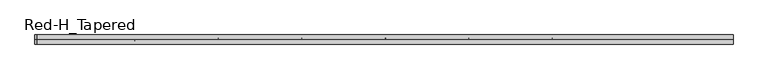
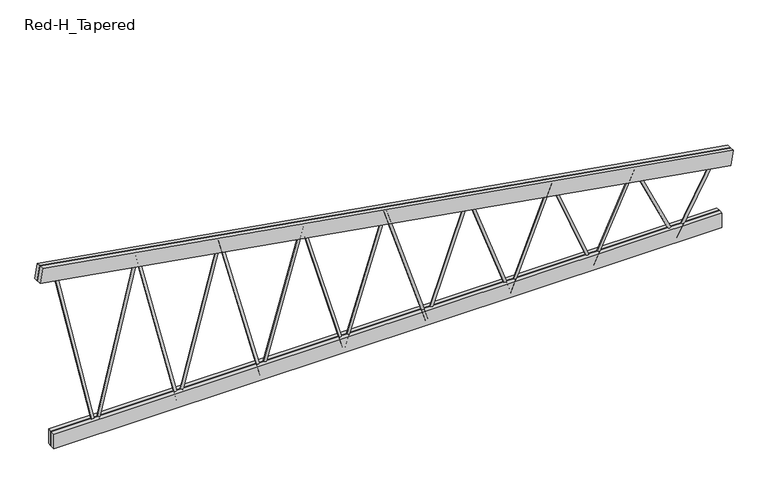
"""IFC4 building model written with IfcOpenShell, lengths in millimetres: beam geometry, Construction_Frames_RedBuilt_Openweb_Red-H_Tapered : Red-H_Tapered."""

from ifc_helpers import new_model, si_unit, point, frame, origin, origin_2d, place, context, project, spatial, polyline, circle_curve, trimmed, segment, composite_curve, outline, extrude, source, transform, mapped, element, save


def red_h_tapered_3aac71cb(model_context):
    return source(origin(), model_context, "Body", "SweptSolid", [
        extrude(outline(composite_curve([segment(trimmed(circle_curve(origin_2d(), 12.7), [point((0.0, -12.7))], [point((0.0, 12.7))], False, "CARTESIAN"), True, "CONTINUOUS"), segment(trimmed(circle_curve(origin_2d(), 12.7), [point((0.0, 12.7))], [point((0.0, -12.7))], False, "CARTESIAN"), True, "CONTINUOUS")], self_intersect=False)), frame((-378.61875, 0.0, -417.8101562), z_axis=(-0.277995532529411, 0.0, 0.9605823670532836), x_axis=(0.0, 1.0, 0.0)), (0.0, 0.0, 1.0), 1361.9598364),
        extrude(outline(composite_curve([segment(trimmed(circle_curve(origin_2d(), 12.7), [point((0.0, 12.7))], [point((0.0, -12.7))], False, "CARTESIAN"), True, "CONTINUOUS"), segment(trimmed(circle_curve(origin_2d(), 12.7), [point((0.0, -12.7))], [point((0.0, 12.7))], False, "CARTESIAN"), True, "CONTINUOUS")], self_intersect=False)), frame((-1135.85625, 0.0, -417.8101562), z_axis=(0.27799553252941006, 0.0, 0.9605823670532838), x_axis=(0.0, 1.0, 0.0)), (0.0, 0.0, 1.0), 1361.9598364),
        extrude(outline(composite_curve([segment(trimmed(circle_curve(origin_2d(), 12.7), [point((0.0, -12.7))], [point((0.0, 12.7000001))], False, "CARTESIAN"), True, "CONTINUOUS"), segment(trimmed(circle_curve(origin_2d(), 12.7), [point((0.0, 12.7000001))], [point((0.0, -12.7))], False, "CARTESIAN"), True, "CONTINUOUS")], self_intersect=False)), frame((-1135.85625, 0.0, -417.8101562), z_axis=(-0.2554865755688276, 0.0, 0.966812603198838), x_axis=(0.0, 1.0, 0.0)), (0.0, 0.0, 1.0), 1481.9516413),
        extrude(outline(composite_curve([segment(trimmed(circle_curve(origin_2d(), 12.7), [point((0.0, 12.7))], [point((0.0, -12.7000001))], False, "CARTESIAN"), True, "CONTINUOUS"), segment(trimmed(circle_curve(origin_2d(), 12.7), [point((0.0, -12.7000001))], [point((0.0, 12.7))], False, "CARTESIAN"), True, "CONTINUOUS")], self_intersect=False)), frame((-1893.09375, 0.0, -417.8101562), z_axis=(0.25548657556883586, 0.0, 0.9668126031988359), x_axis=(0.0, 1.0, 0.0)), (0.0, 0.0, 1.0), 1481.9516413),
        extrude(outline(composite_curve([segment(trimmed(circle_curve(origin_2d(), 12.7), [point((0.0, -12.7))], [point((0.0, 12.7))], False, "CARTESIAN"), True, "CONTINUOUS"), segment(trimmed(circle_curve(origin_2d(), 12.7), [point((0.0, 12.7))], [point((0.0, -12.7))], False, "CARTESIAN"), True, "CONTINUOUS")], self_intersect=False)), frame((-1893.09375, 0.0, -417.8101562), z_axis=(-0.23624830304325084, 0.0, 0.9716927185634275), x_axis=(0.0, 1.0, 0.0)), (0.0, 0.0, 1.0), 1602.6305591),
        extrude(outline(composite_curve([segment(trimmed(circle_curve(origin_2d(), 12.7), [point((0.0, 12.7))], [point((0.0, -12.7))], False, "CARTESIAN"), True, "CONTINUOUS"), segment(trimmed(circle_curve(origin_2d(), 12.7), [point((0.0, -12.7))], [point((0.0, 12.7))], False, "CARTESIAN"), True, "CONTINUOUS")], self_intersect=False)), frame((-2650.33125, 0.0, -417.8101562), z_axis=(0.23624830304324398, 0.0, 0.9716927185634292), x_axis=(0.0, 1.0, 0.0)), (0.0, 0.0, 1.0), 1602.6305591),
        extrude(outline(composite_curve([segment(trimmed(circle_curve(origin_2d(), 12.7), [point((0.0, -12.7))], [point((0.0, 12.7))], False, "CARTESIAN"), True, "CONTINUOUS"), segment(trimmed(circle_curve(origin_2d(), 12.7), [point((0.0, 12.7))], [point((0.0, -12.7))], False, "CARTESIAN"), True, "CONTINUOUS")], self_intersect=False)), frame((-2650.33125, 0.0, -417.8101562), z_axis=(-0.21963526223165897, 0.0, 0.9755820578426145), x_axis=(0.0, 1.0, 0.0)), (0.0, 0.0, 1.0), 1723.8522911),
        extrude(outline(composite_curve([segment(trimmed(circle_curve(origin_2d(), 12.7), [point((0.0, -12.7))], [point((0.0, 12.7))], False, "CARTESIAN"), True, "CONTINUOUS"), segment(trimmed(circle_curve(origin_2d(), 12.7), [point((0.0, 12.7))], [point((0.0, -12.7))], False, "CARTESIAN"), True, "CONTINUOUS")], self_intersect=False)), frame((2650.33125, 0.0, -417.8101562), z_axis=(0.48331839774277513, 0.0, 0.8754446449681195), x_axis=(0.0, 1.0, 0.0)), (0.0, 0.0, 1.0), 783.3733451),
        extrude(outline(composite_curve([segment(trimmed(circle_curve(origin_2d(), 12.7), [point((0.0, 12.7))], [point((0.0, -12.7))], False, "CARTESIAN"), True, "CONTINUOUS"), segment(trimmed(circle_curve(origin_2d(), 12.7), [point((0.0, -12.7))], [point((0.0, 12.7))], False, "CARTESIAN"), True, "CONTINUOUS")], self_intersect=False)), frame((2650.33125, 0.0, -417.8101562), z_axis=(-0.4233271479189003, 0.0, 0.9059768903426011), x_axis=(0.0, 1.0, 0.0)), (0.0, 0.0, 1.0), 894.3880681),
        extrude(outline(composite_curve([segment(trimmed(circle_curve(origin_2d(), 12.7), [point((0.0, -12.7))], [point((0.0, 12.7))], False, "CARTESIAN"), True, "CONTINUOUS"), segment(trimmed(circle_curve(origin_2d(), 12.7), [point((0.0, 12.7))], [point((0.0, -12.7))], False, "CARTESIAN"), True, "CONTINUOUS")], self_intersect=False)), frame((1893.09375, 0.0, -417.8101562), z_axis=(0.42332714791889964, 0.0, 0.9059768903426014), x_axis=(0.0, 1.0, 0.0)), (0.0, 0.0, 1.0), 894.3880681),
        extrude(outline(composite_curve([segment(trimmed(circle_curve(origin_2d(), 12.7), [point((0.0, 12.7))], [point((0.0, -12.7))], False, "CARTESIAN"), True, "CONTINUOUS"), segment(trimmed(circle_curve(origin_2d(), 12.7), [point((0.0, -12.7))], [point((0.0, 12.7))], False, "CARTESIAN"), True, "CONTINUOUS")], self_intersect=False)), frame((1893.09375, 0.0, -417.8101562), z_axis=(-0.3754069541599523, 0.0, 0.9268600858642838), x_axis=(0.0, 1.0, 0.0)), (0.0, 0.0, 1.0), 1008.5555044),
        extrude(outline(composite_curve([segment(trimmed(circle_curve(origin_2d(), 12.7), [point((0.0, -12.7))], [point((0.0, 12.7))], False, "CARTESIAN"), True, "CONTINUOUS"), segment(trimmed(circle_curve(origin_2d(), 12.7), [point((0.0, 12.7))], [point((0.0, -12.7))], False, "CARTESIAN"), True, "CONTINUOUS")], self_intersect=False)), frame((1135.85625, 0.0, -417.8101562), z_axis=(0.37540695415995146, 0.0, 0.9268600858642841), x_axis=(0.0, 1.0, 0.0)), (0.0, 0.0, 1.0), 1008.5555044),
        extrude(outline(composite_curve([segment(trimmed(circle_curve(origin_2d(), 12.7), [point((0.0, 12.7))], [point((0.0, -12.7))], False, "CARTESIAN"), True, "CONTINUOUS"), segment(trimmed(circle_curve(origin_2d(), 12.7), [point((0.0, -12.7))], [point((0.0, 12.7))], False, "CARTESIAN"), True, "CONTINUOUS")], self_intersect=False)), frame((1135.85625, 0.0, -417.8101562), z_axis=(-0.3365750833372033, 0.0, 0.9416566323647674), x_axis=(0.0, 1.0, 0.0)), (0.0, 0.0, 1.0), 1124.9161591),
        extrude(outline(composite_curve([segment(trimmed(circle_curve(origin_2d(), 12.7), [point((0.0, -12.7))], [point((0.0, 12.7))], False, "CARTESIAN"), True, "CONTINUOUS"), segment(trimmed(circle_curve(origin_2d(), 12.7), [point((0.0, 12.7))], [point((0.0, -12.7))], False, "CARTESIAN"), True, "CONTINUOUS")], self_intersect=False)), frame((378.61875, 0.0, -417.8101562), z_axis=(0.33657508333720376, 0.0, 0.9416566323647673), x_axis=(0.0, 1.0, 0.0)), (0.0, 0.0, 1.0), 1124.9161591),
        extrude(outline(composite_curve([segment(trimmed(circle_curve(origin_2d(), 12.7), [point((0.0, 12.7))], [point((0.0, -12.6999999))], False, "CARTESIAN"), True, "CONTINUOUS"), segment(trimmed(circle_curve(origin_2d(), 12.7), [point((0.0, -12.6999999))], [point((0.0, 12.7))], False, "CARTESIAN"), True, "CONTINUOUS")], self_intersect=False)), frame((378.61875, 0.0, -417.8101562), z_axis=(-0.3046365038173337, 0.0, 0.952468687433845), x_axis=(0.0, 1.0, 0.0)), (0.0, 0.0, 1.0), 1242.8541729),
        extrude(outline(composite_curve([segment(trimmed(circle_curve(origin_2d(), 12.7), [point((0.0, 12.6999999))], [point((0.0, -12.7))], False, "CARTESIAN"), True, "CONTINUOUS"), segment(trimmed(circle_curve(origin_2d(), 12.7), [point((0.0, -12.7))], [point((0.0, 12.6999999))], False, "CARTESIAN"), True, "CONTINUOUS")], self_intersect=False)), frame((-378.61875, 0.0, -417.8101562), z_axis=(0.30463650381731205, 0.0, 0.952468687433852), x_axis=(0.0, 1.0, 0.0)), (0.0, 0.0, 1.0), 1242.8541729),
        extrude(outline(polyline([(-3054.35, 41.275), (3054.35, 41.275), (3054.35, 3.175), (-3054.35, 3.175), (-3054.35, 41.275)])), frame((0.0, 0.0, -436.8601562), z_axis=(0.0, 0.0, 1.0), x_axis=(1.0, 0.0, 0.0)), (0.0, 0.0, 1.0), 139.7),
        extrude(outline(polyline([(-3054.35, -3.175), (3054.35, -3.175), (3054.35, -41.275), (-3054.35, -41.275), (-3054.35, -3.175)])), frame((0.0, 0.0, -436.8601562), z_axis=(0.0, 0.0, 1.0), x_axis=(1.0, 0.0, 0.0)), (0.0, 0.0, 1.0), 139.7),
        extrude(outline(polyline([(0.0, 38.1), (6401.4173313, 38.1), (6401.4173313, 0.0), (0.0, 0.0), (0.0, 38.1)])), frame((-3179.231088, 3.175, 1203.3934066), z_axis=(0.1666505938890901, 0.0, 0.9860160138437984), x_axis=(0.9860160138437984, 0.0, -0.1666505938890901)), (0.0, 0.0, 1.0), 139.7),
        extrude(outline(polyline([(0.0, 38.1), (6401.4173313, 38.1), (6401.4173313, 0.0), (0.0, 0.0), (0.0, 38.1)])), frame((-3179.231088, -41.275, 1203.3934066), z_axis=(0.1666505938890901, 0.0, 0.9860160138437984), x_axis=(0.9860160138437984, 0.0, -0.1666505938890901)), (0.0, 0.0, 1.0), 139.7),
    ])


if __name__ == "__main__":
    model = new_model("IFC4")
    model_context = context("Model", 3, world=origin())
    ifc_project = project(units=[si_unit("LENGTHUNIT", "METRE", prefix="MILLI")], contexts=[model_context])
    site = spatial("IfcSite", under=ifc_project)
    building = spatial("IfcBuilding", under=site)
    placement = place(None, origin())
    red_h_tapered_shape = red_h_tapered_3aac71cb(model_context)
    element("IfcBeam", 1, ObjectType="Construction_Frames_RedBuilt_Openweb_Red-H_Tapered : Red-H_Tapered", at=placement, inside=building, context=model_context, shape_type="MappedRepresentation", body=[
        mapped(red_h_tapered_shape, transform((0.0, 0.0, 0.0), x_axis=(1.0, 0.0, 0.0), y_axis=(0.0, 1.0, 0.0), z_axis=(0.0, 0.0, 1.0))),
    ])
    save(model, "model.ifc")

# Revit data of these elements
# Type "Construction_Frames_RedBuilt_Openweb_Red-H_Tapered : Red-H_Tapered"
#   Youtube clip = ""
#   Weight Net (Kg) = "0"
#   Webs = "Up to 2\" diameter tubular steel"
#   Uniformat II Description = ""
#   Uniformat II Code = ""
#   Uniclass 2015 Name = "Softwood trusses"
#   Uniclass 2015 Code = "Pr_20_85_90_81"
#   Uniclass 2.0 Description = "Structural Framing Systems"
#   Uniclass 2.0 Code = "SS-15-10-75"
#   Uniclass 1.4 Description = "Trusses"
#   Uniclass 1.4 Code = "L3523"
#   UNSPSC Code = "30103606"
#   Technical description = "http://www.redbuilt.com/reference/literature-and-other-resources"
#   Region South America = "None"
#   Region Oceania = "None"
#   Region North America = "US"
#   Region Middle East = "None"
#   Region Europe = "None"
#   Region Asia = "None"
#   Region Antarctica = "None"
#   Region Africa = "None"
#   QR code = "http://bimobject.com/redbuilt/product/redbuilt-0003"
#   Product url = "http://www.redbuilt.com/products/default.aspx?id=2"
#   Product group = "Wood Trusses"
#   Product family = "Construction"
#   Product data url = "https://bimobject.com/redbuilt/product/redbuilt-0003"
#   Product certification = ""
#   Product SKU = "redbuilt-0003"
#   Product Page URL = "http://www.redbuilt.com/commercial-systems/red-m-red-h-open-web-trusses"
#   Product Guid = "2c5793f2-6ffb-4665-b825-cf90c048e711"
#   Product Documentation Link = "http://www.redbuilt.com/documents/OW_Guide_2017_07_LowRes_wLinks.pdf"
#   OmniClass Description = "Wood Trusses"
#   OmniClass Code = "23-13 35 19 13 17"
#   NBS Reference Description = ""
#   NBS Reference Code = ""
#   Material secondary = "Steel"
#   Material main = "CHARRED WOOD"
#   Masterformat 2014 Description = "Metal-Web Wood Joists"
#   Masterformat 2014 Code = "06 17 36"
#   Manufacturer name = "RedBuilt"
#   Manufacturer country = "United States"
#   Installation instructions = "http://www.redbuilt.com/documents/Installation_Sheets_Open-Web.pdf"
#   IFC Classification = ""
#   EAN code = ""
#   Design country = "United States"
#   Product Information = "http://redbuilt.com/products/default.aspx?id=2"
#   Model = "Red-H-Tapered"
#   Manufacturer URL = "http://redbuilt.com/"
#   Manufacturer = "RedBuilt™"
#   Description = "Open Web Truss"
#   Date of publishing = "8/17/2010"
#   Contact us = "http://redbuilt.com/contact/"
#   Chords = "Double 1½\" x 5½\" MSR lumber"
#   COBIe Type Category = ""
#   Brand url = "http://www.redbuilt.com"
#   BIMobject main category code = "construction"
#   BIMobject main category = "Construction"
#   BIMobject category code = "construction-frames-trusses"
#   BIMobject category = "Frames & Trusses"
#   Web Radius = 0' - 0 1/2"
#   Web Layout Offset Start [instance default] = 0' - 5"
#   Web Layout Offset End [instance default] = 0' - 5"
#   Web Diameter = 0' - 1"
#   TotalLength [instance default] = 20' - 0"
#   Span Minimum = 4' - 0"
#   Span Maximum = 70' - 0"
#   Span Limit [instance default] = 20' - 0"
#   Nominal width = 0' - 0"
#   Nominal height = 0' - 0"
#   Inner Depth Top [instance default] = 0' - 2.76372"
#   Depth Start [instance default] = 6' - 0"
#   Top Chord Length [instance default] = 20' - 1.19701"
#   TC Extension Start Aux [instance default] = 0' - 0"
#   TC Extension End Aux [instance default] = 0' - 0"
#   T-B Chord Length Difference L [instance default] = 0' - 4"
#   T-B Chord Length Difference [instance default] = 0' - 4"
#   Height 2 [instance default] = 6' - 0"
#   Depth Minimum at Wall = 2' - 0"
#   Depth Maximum at Wall = 6' - 0"
#   Depth Lower End [instance default] = 2' - 0"
#   Depth Higher End [instance default] = 6' - 0"
#   Depth End [instance default] = 2' - 0"
#   Depth 2 [instance default] = 2' - 0"
#   Chord Width = 0' - 3 1/4"
#   Chord Thickness = 0' - 1 1/2"
#   Chord Depth = 0' - 5 1/2"
#   Offset Start [instance default] = 0' - 0"
#   TC Extension Start [instance default] = 0' - 0"
#   End Panel = 0' - 5"
#   Offset End [instance default] = 0' - 0"
#   TC Extension End [instance default] = 0' - 0"
#   Length [instance default] = 20' - 0"
#   Angle [instance default] = 5.71059°
#   Span Limit Warning [instance default] = no
#   Edition number = 1
#   Top Bearing Start [instance default] = yes
#   Top Bearing End [instance default] = yes
#   Bottom Bearing Start [instance default] = no
#   Bottom Bearing End [instance default] = no
#   8 Panels [instance default] = yes
#   16 Panels [instance default] = no
#   12 Panels [instance default] = no
#   Web Material = RedBuilt-Steel, Galvanized
#   Clip Material = RedBuilt-Steel, Galvanized
#   Chords Material = WOOD-OAKFIRE
#   URL = ""
#   Assembly Code = ""
# Element 1 (IfcBeam, "Construction_Frames_RedBuilt_Openweb_Red-H_Tapered : Red-H_Tapered")
#   TotalLength = 20' - 8 1/2"
#   Span Limit = 20' - 8 1/2"
#   Inner Depth Top = 0' - 2.789"
#   Depth Start = 5' - 0"
#   Top Chord Length = 21' - 0.0243"
#   Height 2 = 5' - 0"
#   Depth Lower End = 2' - 4"
#   Depth Higher End = 5' - 0"
#   Depth End = 2' - 4"
#   Depth 2 = 3' - 6"
#   Angle = 9.59313°
#   Materials on its faces: "RedBuilt-Steel, Galvanized", "WOOD-OAKFIRE"
# Materials
#   "RedBuilt-Steel, Galvanized": class "Metal", colour RGB 164 172 176, transparency 0, Manufacturer = "RedBuilt. LLC", Comments = "Openweb Metal Web", URL = "http://www.redbuilt.com/", Description = "Galvanized steel", Cost = 0
#   "WOOD-OAKFIRE": class "Wood", colour RGB 198 202 183, transparency 0, Description = "Generic wood", Cost = 0
